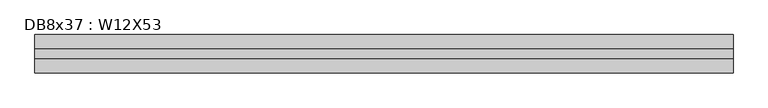
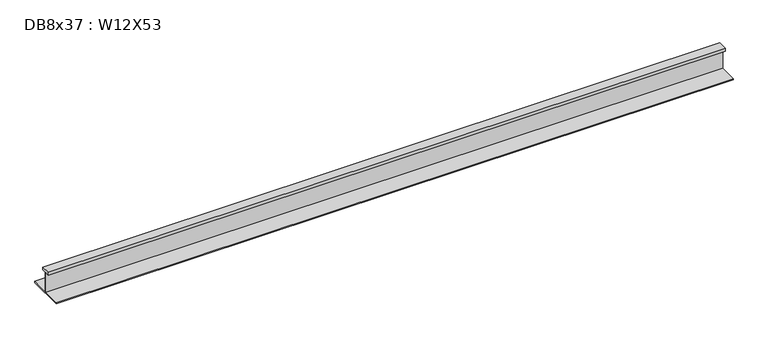
"""IFC4 building model written with IfcOpenShell, lengths in millimetres: beam geometry, DB8x37 : W12X53."""

from ifc_helpers import new_model, si_unit, frame, origin, place, context, project, spatial, polyline, outline, extrude, source, transform, mapped, element, save


def db8x37_w12x53_959fe51c(model_context):
    return source(origin(), model_context, "Body", "SweptSolid", [
        extrude(outline(polyline([(38.1, 145.415), (38.1, 120.015), (2.921, 120.015), (2.921, -48.4505), (152.4, -48.4505), (152.4, -58.1025), (-152.4, -58.1025), (-152.4, -48.4505), (-2.921, -48.4505), (-2.921, 120.015), (-38.1, 120.015), (-38.1, 145.415), (38.1, 145.415)])), frame((-2832.0999994, 0.0, 0.0), z_axis=(1.0, 0.0, 0.0), x_axis=(0.0, 1.0, 0.0)), (0.0, 0.0, 1.0), 5540.6289994),
    ])


if __name__ == "__main__":
    model = new_model("IFC4")
    model_context = context("Model", 3, world=origin())
    ifc_project = project(units=[si_unit("LENGTHUNIT", "METRE", prefix="MILLI")], contexts=[model_context])
    site = spatial("IfcSite", under=ifc_project)
    building = spatial("IfcBuilding", under=site)
    placement = place(None, origin())
    db8x37_w12x53_shape = db8x37_w12x53_959fe51c(model_context)
    element("IfcBeam", 1, ObjectType="DB8x37 : W12X53", at=placement, inside=building, context=model_context, shape_type="MappedRepresentation", body=[
        mapped(db8x37_w12x53_shape, transform((0.0, 0.0, 0.0), x_axis=(1.0, 0.0, 0.0), y_axis=(0.0, 1.0, 0.0), z_axis=(0.0, 0.0, 1.0))),
    ])
    save(model, "model.ifc")

# Revit data of these elements
# Type "DB8x37 : W12X53"
#   Assembly Code = "B10"
#   W = 53
#   Length [instance default] = 5' - 0"
#   bf = 0' - 10"
#   d = 1' - 0.1"
#   k = 0' - 1 3/8"
#   k2 = 0' - 0.8"
#   tf = 0' - 0.575"
#   tw = 0' - 0.345"
#   A = 0.108333 SF
#   Structural Material [instance default] = Steel ASTM A992
# Element 1 (IfcBeam, "DB8x37 : W12X53")
#   Materials on its faces: "Steel ASTM A992"
# Materials
#   "Steel ASTM A992": class "Metal", colour RGB 199 199 199, transparency 0, Description = "Structural steel 50ksi", Cost = 0
